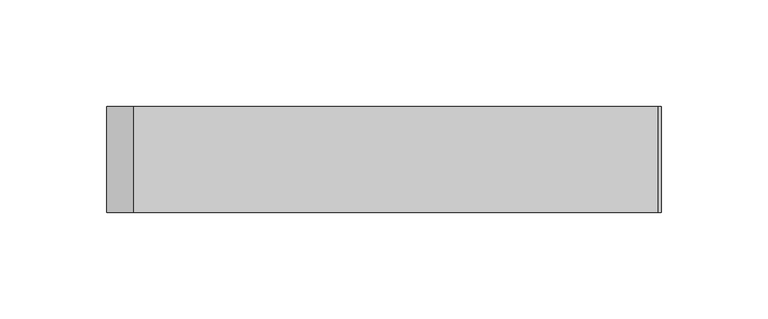
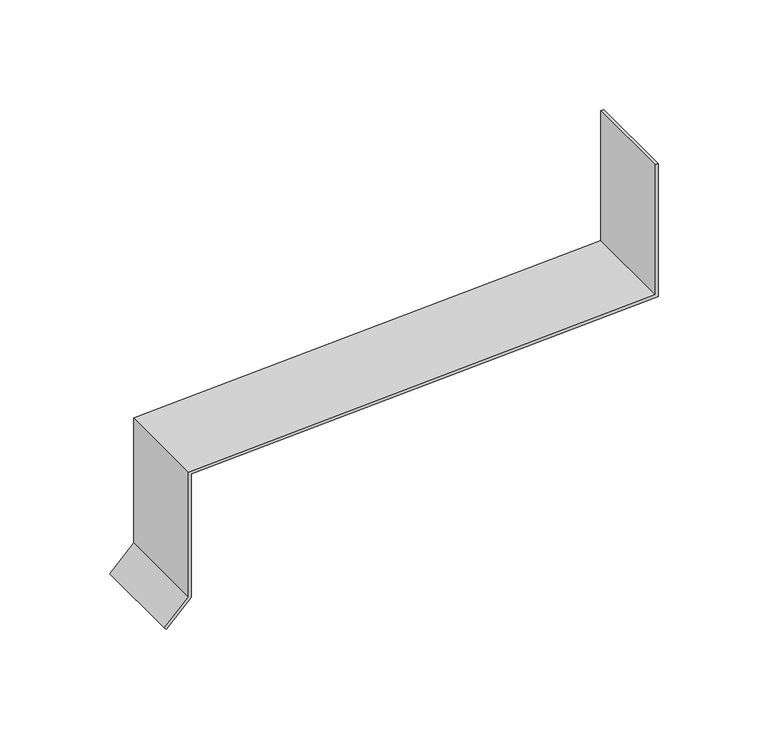
"""IFC4 building model written with IfcOpenShell, lengths in millimetres: proxy geometry, Generic Models 7:Generic Models 1:5:Generic Models 1:5 : Generic Models 7:Generic Models 1:337419:19 : Generic Models 7:Generic Models 1:5:Generic Models 1:5 : Generic Models 7:Generic Models 1:337419:311462."""

from ifc_helpers import new_model, si_unit, origin, place, context, project, spatial, faceted_brep, source, transform, mapped, element, save


def generic_models_70099b53(model_context):
    return source(origin(), model_context, "Body", "Brep", [
        faceted_brep([(667548.8992239, -568236.4915363, 6180.8221905), (667548.8992239, -568236.4915363, 6182.4118691), (667548.8992239, -568236.4915363, 6254.75), (667547.3117239, -568236.4915363, 6254.75), (667547.3117239, -568236.4915363, 6182.3286718), (667301.2492239, -568236.4915363, 6169.4330826), (667301.2492239, -568236.4915363, 6099.8348677), (667288.5492239, -568236.4915363, 6087.1348677), (667289.6717559, -568236.4915363, 6086.0123357), (667302.8367239, -568236.4915363, 6099.1773037), (667302.8367239, -568236.4915363, 6167.9266014), (667548.8992239, -568186.6413841, 6180.8221905), (667302.8367239, -568186.6413841, 6167.9266014), (667302.8367239, -568186.6413841, 6099.1773037), (667289.6717559, -568186.6413841, 6086.0123357), (667288.5492239, -568186.6413841, 6087.1348677), (667301.2492239, -568186.6413841, 6099.8348677), (667301.2492239, -568186.6413841, 6167.843404), (667301.2492239, -568186.6413841, 6169.4330826), (667547.3117239, -568186.6413841, 6182.3286718), (667547.3117239, -568186.6413841, 6254.75), (667548.8992239, -568186.6413841, 6254.75), (667548.8992239, -568233.850616, 6180.8221905)], [[[0, 1, 2, 3, 4, 5, 6, 7, 8, 9, 10]], [[11, 12, 13, 14, 15, 16, 17, 18, 19, 20, 21]], [[4, 3, 20, 19]], [[0, 10, 12, 11, 22]], [[10, 9, 13, 12]], [[9, 8, 14, 13]], [[8, 7, 15, 14]], [[7, 6, 16, 15]], [[6, 5, 18, 17, 16]], [[5, 4, 19, 18]], [[2, 1, 0, 22, 11, 21]], [[3, 2, 21, 20]]]),
    ])


if __name__ == "__main__":
    model = new_model("IFC4")
    model_context = context("Model", 3, world=origin())
    ifc_project = project(units=[si_unit("LENGTHUNIT", "METRE", prefix="MILLI")], contexts=[model_context])
    site = spatial("IfcSite", under=ifc_project)
    building = spatial("IfcBuilding", under=site)
    placement = place(None, origin())
    generic_models_shape = generic_models_70099b53(model_context)
    element("IfcBuildingElementProxy", 1, Name="Generic Models 7:Generic Models 1:5:Generic Models 1:5 : Generic Models 7:Generic Models 1:337419:19 : Generic Models 7:Generic Models 1:5:Generic Models 1:5 : Generic Models 7:Generic Models 1:337419:311462", ObjectType="Generic Models 7:Generic Models 1:5:Generic Models 1:5 : Generic Models 7:Generic Models 1:337419:19 : Generic Models 7:Generic Models 1:5:Generic Models 1:5 : Generic Models 7:Generic Models 1:337419:311462", at=placement, inside=building, context=model_context, shape_type="MappedRepresentation", body=[
        mapped(generic_models_shape, transform((0.0, 0.0, 0.0), x_axis=(1.0, 0.0, 0.0), y_axis=(0.0, 1.0, 0.0), z_axis=(0.0, 0.0, 1.0))),
    ])
    save(model, "model.ifc")

# Revit data of these elements
# Type "Generic Models 7:Generic Models 1:5:Generic Models 1:5 : Generic Models 7:Generic Models 1:337419:19 : Generic Models 7:Generic Models 1:5:Generic Models 1:5 : Generic Models 7:Generic Models 1:337419:311462"
#   NameOverride = "Generic Models 7:Generic Models 1:5:Generic Models 1:5 : Generic Models 7:Generic Models 1:337419:311462"
#   ObjectTypeOverride = "Generic Models 1:5 : Generic Models 7:Generic Models 1:337419"
#   Reference = "Generic Models 1"
#   Tag = "311462"
# Element 1 (IfcBuildingElementProxy, "Generic Models 7:Generic Models 1:5:Generic Models 1:5 : Generic Models 7:Generic Models 1:337419:19 : Generic Models 7:Generic Models 1:5:Generic Models 1:5 : Generic Models 7:Generic Models 1:337419:311462")
#   Materials on its faces: "SLOPED SHEET METAL COPING - (COLOR TO MATCH RESIN PANEL)"
# Materials
#   "SLOPED SHEET METAL COPING - (COLOR TO MATCH RESIN PANEL)": class "Generic", colour RGB 240 240 240, transparency 0, Keynote = "M07711300.01", Cost = 0
